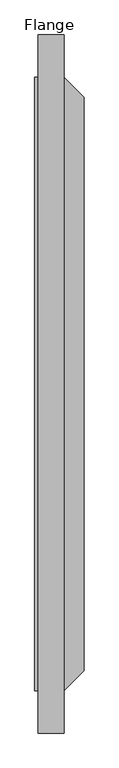
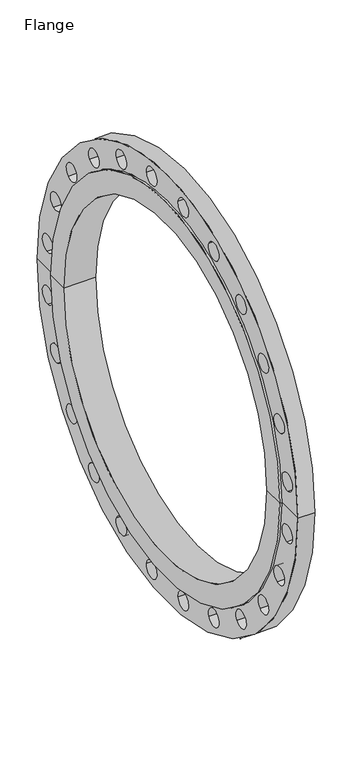
"""IFC4 building model written with IfcOpenShell, lengths in millimetres: proxy geometry, Flange : CASTED FLANGE PN16."""

import ifcopenshell
import ifcopenshell.guid

model = None  # the IFC model being written
_history = None  # IfcOwnerHistory: only IFC2X3 demands one
_inside = {}  # id of a spatial element -> (the spatial element, [elements in it])
_under = {}  # id of a project, library or spatial element -> (it, [spatial elements below it])
_declared = {}  # id of a project -> (the project, [libraries it declares])
_typed = {}  # id of a type object -> (the type object, [elements of that type])
_made_of = {}  # id of a material, layer set ... -> (it, [elements and type objects made of it])


def new_model(schema):
    """Start an empty IFC model of exactly this schema.

    Asked for "IFC4X3", IfcOpenShell would pick the latest addendum, in which some entities
    have other attributes; the version numbers below select the first issue.
    IFC2X3 requires an IfcOwnerHistory on every rooted entity: one is made here for all.
    """
    global model, _history
    if schema == "IFC4X3":
        model = ifcopenshell.file(schema_version=(4, 3, 0, 0))
    else:
        model = ifcopenshell.file(schema=schema)
    _inside.clear()
    _under.clear()
    _declared.clear()
    _typed.clear()
    _made_of.clear()
    _history = None
    if model.schema == "IFC2X3":
        org = make("IfcOrganization", Name="unknown")
        user = make(
            "IfcPersonAndOrganization",
            ThePerson=make("IfcPerson", FamilyName="unknown"),
            TheOrganization=org,
        )
        app = make(
            "IfcApplication",
            ApplicationDeveloper=org,
            Version="unknown",
            ApplicationFullName="unknown",
            ApplicationIdentifier="unknown",
        )
        _history = make(
            "IfcOwnerHistory",
            OwningUser=user,
            OwningApplication=app,
            ChangeAction="ADDED",
            CreationDate=0,
        )
    return model


def make(cls, **values):
    """One entity of the class cls with the attributes given. An attribute that is None is left unset."""
    return model.create_entity(
        cls, **{name: value for name, value in values.items() if value is not None}
    )


def rooted(cls, **values):
    """An entity with a GlobalId (a new one), such as an element, a storey or a relation."""
    return make(cls, GlobalId=ifcopenshell.guid.new(), OwnerHistory=_history, **values)


def si_unit(unit_type, name, prefix=None):
    """IfcSIUnit, for example si_unit("LENGTHUNIT", "METRE", prefix="MILLI")."""
    return make("IfcSIUnit", UnitType=unit_type, Prefix=prefix, Name=name)


def assignment(units):
    """IfcUnitAssignment: the units of a project."""
    return None if units is None else make("IfcUnitAssignment", Units=units)


def point(xyz):
    """IfcCartesianPoint."""
    return None if xyz is None else make("IfcCartesianPoint", Coordinates=xyz)


def direction(xyz):
    """IfcDirection."""
    return None if xyz is None else make("IfcDirection", DirectionRatios=xyz)


def frame(location, z_axis=None, x_axis=None):
    """IfcAxis2Placement3D, a coordinate frame: its origin and axes. An axis left out is left unset."""
    return make(
        "IfcAxis2Placement3D",
        Location=point(location),
        Axis=direction(z_axis),
        RefDirection=direction(x_axis),
    )


def origin():
    """The frame at (0, 0, 0) with its axes left unset."""
    return frame((0.0, 0.0, 0.0))


def place(relative_to, where):
    """IfcLocalPlacement: puts the frame where relative to a parent placement (None: the world)."""
    return make(
        "IfcLocalPlacement", PlacementRelTo=relative_to, RelativePlacement=where
    )


def context(
    kind, dimensions, precision=None, world=None, true_north=None, identifier=None
):
    """IfcGeometricRepresentationContext, for example the 3D "Model" context."""
    return make(
        "IfcGeometricRepresentationContext",
        ContextIdentifier=identifier,
        ContextType=kind,
        CoordinateSpaceDimension=dimensions,
        Precision=precision,
        WorldCoordinateSystem=world,
        TrueNorth=true_north,
    )


def project(units=None, contexts=None):
    """IfcProject with its units and contexts."""
    return rooted(
        "IfcProject",
        Name="project",
        RepresentationContexts=contexts,
        UnitsInContext=assignment(units),
    )


def spatial(cls, under=None, at=None, **own):
    """A site, building, storey or space (cls), placed at a placement, below another one or the project."""
    s = rooted(cls, ObjectPlacement=at, **own)
    if under is not None:
        _under.setdefault(under.id(), (under, []))[1].append(s)
    return s


def polyline(points):
    """IfcPolyline through the points."""
    return make("IfcPolyline", Points=[point(p) for p in points])


def circle_curve(where, radius):
    """IfcCircle in the frame where."""
    return make("IfcCircle", Position=where, Radius=radius)


def shape(context_of_items, identifier, shape_type, items):
    """IfcShapeRepresentation: the items that make up one representation, for example the "Body"."""
    return make(
        "IfcShapeRepresentation",
        ContextOfItems=context_of_items,
        RepresentationIdentifier=identifier,
        RepresentationType=shape_type,
        Items=items,
    )


def source(mapping_origin, context_of_items, identifier, shape_type, items):
    """IfcRepresentationMap: a shape defined once, which mapped items show again and again."""
    return make(
        "IfcRepresentationMap",
        MappingOrigin=mapping_origin,
        MappedRepresentation=shape(context_of_items, identifier, shape_type, items),
    )


def transform(
    local_origin,
    x_axis=None,
    y_axis=None,
    z_axis=None,
    scale=None,
    scale2=None,
    scale3=None,
    uniform=True,
):
    """IfcCartesianTransformationOperator3D, or its non-uniform kind. x_axis, y_axis, z_axis: its Axis1, 2, 3."""
    if uniform:
        return make(
            "IfcCartesianTransformationOperator3D",
            Axis1=direction(x_axis),
            Axis2=direction(y_axis),
            LocalOrigin=point(local_origin),
            Scale=scale,
            Axis3=direction(z_axis),
        )
    return make(
        "IfcCartesianTransformationOperator3DnonUniform",
        Axis1=direction(x_axis),
        Axis2=direction(y_axis),
        LocalOrigin=point(local_origin),
        Scale=scale,
        Axis3=direction(z_axis),
        Scale2=scale2,
        Scale3=scale3,
    )


def mapped(mapping_source, mapping_target):
    """IfcMappedItem: shows the shape of a source again, moved by a transform."""
    return make(
        "IfcMappedItem", MappingSource=mapping_source, MappingTarget=mapping_target
    )


def made_of(thing, what):
    """Note that an element or type object is made of a material, layer set ...; save() writes the relation."""
    if what is not None:
        _made_of.setdefault(what.id(), (what, []))[1].append(thing)
    return thing


def element(
    cls,
    number,
    at=None,
    inside=None,
    cuts=None,
    type_object=None,
    material=None,
    context=None,
    identifier="Body",
    shape_type=None,
    held_by="IfcProductDefinitionShape",
    body=None,
    shapes=None,
    **own,
):
    """One element of the class cls, such as IfcWall. Its Tag is "e" and its number.

    at: its placement. inside: the storey or other place that contains it. cuts: it is an
    opening in that element (IfcRelVoidsElement). A single representation is given by context,
    identifier, shape_type and body (its items); several are given by shapes. held_by: the class
    of the entity that holds the representations. save() writes the other relations.
    """
    e = rooted(cls, Tag="e%d" % number, ObjectPlacement=at, **own)
    if body is not None:
        shapes = [shape(context, identifier, shape_type, body)]
    if shapes is not None:
        e.Representation = make(held_by, Representations=shapes)
    if inside is not None:
        _inside.setdefault(inside.id(), (inside, []))[1].append(e)
    if cuts is not None:
        rooted(
            "IfcRelVoidsElement", RelatingBuildingElement=cuts, RelatedOpeningElement=e
        )
    if type_object is not None:
        _typed.setdefault(type_object.id(), (type_object, []))[1].append(e)
    return made_of(e, material)


def aggregate(whole, parts):
    """IfcRelAggregates: a whole, such as a stair, and the parts it consists of."""
    return rooted("IfcRelAggregates", RelatingObject=whole, RelatedObjects=parts)


def save(model, path):
    """Write the relations noted so far, then the file.

    IfcRelAggregates (storeys below a building ...), IfcRelContainedInSpatialStructure (elements
    in a storey), IfcRelDefinesByType, IfcRelAssociatesMaterial and IfcRelDeclares: one each for
    every whole, place, type object, material and project.
    """
    for whole, parts in _under.values():
        aggregate(whole, parts)
    for where, things in _inside.values():
        rooted(
            "IfcRelContainedInSpatialStructure",
            RelatedElements=things,
            RelatingStructure=where,
        )
    for kind, things in _typed.values():
        rooted("IfcRelDefinesByType", RelatedObjects=things, RelatingType=kind)
    for what, things in _made_of.values():
        rooted("IfcRelAssociatesMaterial", RelatedObjects=things, RelatingMaterial=what)
    for by, libraries in _declared.values():
        rooted("IfcRelDeclares", RelatingContext=by, RelatedDefinitions=libraries)
    model.write(path)


def plane_surface(at):
    """IfcPlane: the flat surface through the origin of the frame at, square to its z axis."""
    return make("IfcPlane", Position=at)


def cylinder_surface(at, radius):
    """IfcCylindricalSurface: all points at the distance radius from the z axis of the frame at."""
    return make("IfcCylindricalSurface", Position=at, Radius=radius)


def revolved_surface(curve, axis_point, axis_direction):
    """IfcSurfaceOfRevolution: the curve turned about the line through axis_point along axis_direction."""
    return make(
        "IfcSurfaceOfRevolution",
        SweptCurve=make("IfcArbitraryOpenProfileDef", ProfileType="CURVE", Curve=curve),
        AxisPosition=make("IfcAxis1Placement", Location=point(axis_point), Axis=direction(axis_direction)),
    )


def advanced_brep(points, edges, surfaces, faces):
    """IfcAdvancedBrep: a solid bounded by faces that lie on surfaces and meet in shared edges.

    An edge is (start, end): straight between two places in points (the first is 0);
    or (start, end, curve); or (start, end, curve, False) where it runs against its curve.
    A face is (place in surfaces, loops), or (place, loops, False) where it looks against
    its surface's normal. A loop lists edges by number (the first is 1), with a minus sign
    where the edge is run from its end to its start. The first loop is the outer one.
    """
    corners = [point(p) for p in points]
    vertices = [make("IfcVertexPoint", VertexGeometry=c) for c in corners]
    made = []
    for start, end, *more in edges:
        made.append(
            make(
                "IfcEdgeCurve",
                EdgeStart=vertices[start],
                EdgeEnd=vertices[end],
                EdgeGeometry=more[0] if more else make("IfcPolyline", Points=[corners[start], corners[end]]),
                SameSense=more[1] if len(more) > 1 else True,
            )
        )
    hull = []
    for where, loops, *sense in faces:
        bounds = []
        for j, loop in enumerate(loops):
            ring = [make("IfcOrientedEdge", EdgeElement=made[abs(k) - 1], Orientation=k > 0) for k in loop]
            bounds.append(
                make(
                    "IfcFaceOuterBound" if j == 0 else "IfcFaceBound",
                    Bound=make("IfcEdgeLoop", EdgeList=ring),
                    Orientation=True,
                )
            )
        hull.append(make("IfcAdvancedFace", Bounds=bounds, FaceSurface=surfaces[where], SameSense=sense[0] if sense else True))
    return make("IfcAdvancedBrep", Outer=make("IfcClosedShell", CfsFaces=hull))


def flange_f2916e97(model_context):
    return source(origin(), model_context, "Body", "AdvancedBrep", [
        advanced_brep(
        [(0.0, 400.0, 0.0), (0.0, 450.5, 0.0), (0.0, -450.5, 0.0), (0.0, -400.0, 0.0), (72.5, 400.0, 0.0), (72.5, -400.0, 0.0), (72.5, 421.0, 0.0), (72.5, -421.0, 0.0), (43.0, 450.5, 0.0), (43.0, -450.5, 0.0), (43.0, 512.5, 0.0), (43.0, -512.5, 0.0), (43.0, -82.324561, -468.2605222), (43.0, -41.6753216, -473.6120961), (43.0, 41.6753216, -473.6120961), (43.0, 82.324561, -468.2605222), (43.0, -200.7141608, -430.9977676), (43.0, -162.8351, -446.6877883), (43.0, -305.4254223, -364.3632273), (43.0, -272.8979353, -389.3224459), (43.0, -389.3224459, -272.8979353), (43.0, -364.3632273, -305.4254223), (43.0, -446.6877883, -162.8351), (43.0, -430.9977676, -200.7141608), (43.0, -473.6120961, -41.6753216), (43.0, -468.2605222, -82.324561), (43.0, 468.2605222, -82.324561), (43.0, 473.6120961, -41.6753216), (43.0, 272.8979353, -389.3224459), (43.0, 305.4254223, -364.3632273), (43.0, 162.8351, -446.6877883), (43.0, 200.7141608, -430.9977676), (43.0, 430.9977676, -200.7141608), (43.0, 446.6877883, -162.8351), (43.0, 364.3632273, -305.4254223), (43.0, 389.3224459, -272.8979353), (43.0, -468.2605222, 82.324561), (43.0, -473.6120961, 41.6753216), (43.0, -272.8979353, 389.3224459), (43.0, -305.4254223, 364.3632273), (43.0, -162.8351, 446.6877883), (43.0, -200.7141608, 430.9977676), (43.0, -41.6753216, 473.6120961), (43.0, -82.324561, 468.2605222), (43.0, 82.324561, 468.2605222), (43.0, 41.6753216, 473.6120961), (43.0, 200.7141608, 430.9977676), (43.0, 162.8351, 446.6877883), (43.0, 305.4254223, 364.3632273), (43.0, 272.8979353, 389.3224459), (43.0, 389.3224459, 272.8979353), (43.0, 364.3632273, 305.4254223), (43.0, 446.6877883, 162.8351), (43.0, 430.9977676, 200.7141608), (43.0, 473.6120961, 41.6753216), (43.0, 468.2605222, 82.324561), (43.0, -430.9977676, 200.7141608), (43.0, -446.6877883, 162.8351), (43.0, -364.3632273, 305.4254223), (43.0, -389.3224459, 272.8979353), (5.0, 512.5, 0.0), (5.0, -512.5, 0.0), (5.0, 450.5, 0.0), (5.0, -450.5, 0.0), (5.0, -41.6753216, -473.6120961), (5.0, -82.324561, -468.2605222), (5.0, 82.324561, -468.2605222), (5.0, 41.6753216, -473.6120961), (5.0, -162.8351, -446.6877883), (5.0, -200.7141608, -430.9977676), (5.0, -272.8979353, -389.3224459), (5.0, -305.4254223, -364.3632273), (5.0, -364.3632273, -305.4254223), (5.0, -389.3224459, -272.8979353), (5.0, -430.9977676, -200.7141608), (5.0, -446.6877883, -162.8351), (5.0, -468.2605222, -82.324561), (5.0, -473.6120961, -41.6753216), (5.0, 473.6120961, -41.6753216), (5.0, 468.2605222, -82.324561), (5.0, 305.4254223, -364.3632273), (5.0, 272.8979353, -389.3224459), (5.0, 200.7141608, -430.9977676), (5.0, 162.8351, -446.6877883), (5.0, 446.6877883, -162.8351), (5.0, 430.9977676, -200.7141608), (5.0, 389.3224459, -272.8979353), (5.0, 364.3632273, -305.4254223), (5.0, -473.6120961, 41.6753216), (5.0, -468.2605222, 82.324561), (5.0, -305.4254223, 364.3632273), (5.0, -272.8979353, 389.3224459), (5.0, -200.7141608, 430.9977676), (5.0, -162.8351, 446.6877883), (5.0, -82.324561, 468.2605222), (5.0, -41.6753216, 473.6120961), (5.0, 41.6753216, 473.6120961), (5.0, 82.324561, 468.2605222), (5.0, 162.8351, 446.6877883), (5.0, 200.7141608, 430.9977676), (5.0, 272.8979353, 389.3224459), (5.0, 305.4254223, 364.3632273), (5.0, 364.3632273, 305.4254223), (5.0, 389.3224459, 272.8979353), (5.0, 430.9977676, 200.7141608), (5.0, 446.6877883, 162.8351), (5.0, 468.2605222, 82.324561), (5.0, 473.6120961, 41.6753216), (5.0, -446.6877883, 162.8351), (5.0, -430.9977676, 200.7141608), (5.0, -389.3224459, 272.8979353), (5.0, -364.3632273, 305.4254223)],
        [
            (0, 1),
            (1, 2, circle_curve(frame((0.0, 0.0, 0.0), z_axis=(-1.0, 0.0, 0.0), x_axis=(0.0, 1.0, 0.0)), 450.5)),
            (2, 3),
            (3, 0, circle_curve(frame((0.0, 0.0, 0.0), z_axis=(1.0, 0.0, 0.0), x_axis=(0.0, 1.0, 0.0)), 400.0)),
            (0, 3, circle_curve(frame((0.0, 0.0, 0.0), z_axis=(1.0, 0.0, 0.0), x_axis=(0.0, 1.0, 0.0)), 400.0)),
            (2, 1, circle_curve(frame((0.0, 0.0, 0.0), z_axis=(-1.0, 0.0, 0.0), x_axis=(0.0, 1.0, 0.0)), 450.5)),
            (4, 0),
            (3, 5),
            (5, 4, circle_curve(frame((72.5, 0.0, 0.0), z_axis=(1.0, 0.0, 0.0), x_axis=(0.0, 1.0, 0.0)), 400.0)),
            (4, 5, circle_curve(frame((72.5, 0.0, 0.0), z_axis=(1.0, 0.0, 0.0), x_axis=(0.0, 1.0, 0.0)), 400.0)),
            (6, 4),
            (5, 7),
            (7, 6, circle_curve(frame((72.5, 0.0, 0.0), z_axis=(1.0, 0.0, 0.0), x_axis=(0.0, 1.0, 0.0)), 421.0)),
            (6, 7, circle_curve(frame((72.5, 0.0, 0.0), z_axis=(1.0, 0.0, 0.0), x_axis=(0.0, 1.0, 0.0)), 421.0)),
            (8, 6),
            (7, 9),
            (9, 8, circle_curve(frame((43.0, 0.0, 0.0), z_axis=(1.0, 0.0, 0.0), x_axis=(0.0, 1.0, 0.0)), 450.5)),
            (8, 9, circle_curve(frame((43.0, 0.0, 0.0), z_axis=(1.0, 0.0, 0.0), x_axis=(0.0, 1.0, 0.0)), 450.5)),
            (10, 8),
            (9, 11),
            (11, 10, circle_curve(frame((43.0, 0.0, 0.0), z_axis=(1.0, 0.0, 0.0), x_axis=(0.0, 1.0, 0.0)), 512.5)),
            (12, 13, circle_curve(frame((43.0, -61.9999413, -470.9363092), z_axis=(-1.0, 0.0, 0.0), x_axis=(0.0, 0.9914448613738129, -0.13052619222003253)), 20.5)),
            (13, 12, circle_curve(frame((43.0, -61.9999413, -470.9363092), z_axis=(-1.0, 0.0, 0.0), x_axis=(0.0, 0.9914448613738129, -0.13052619222003253)), 20.5)),
            (14, 15, circle_curve(frame((43.0, 61.9999413, -470.9363092), z_axis=(-1.0, 0.0, 0.0), x_axis=(0.0, 0.9914448613738089, 0.13052619222006298)), 20.5)),
            (15, 14, circle_curve(frame((43.0, 61.9999413, -470.9363092), z_axis=(-1.0, 0.0, 0.0), x_axis=(0.0, 0.9914448613738089, 0.13052619222006298)), 20.5)),
            (16, 17, circle_curve(frame((43.0, -181.7746304, -438.8427779), z_axis=(-1.0, 0.0, 0.0), x_axis=(0.0, 0.9238795325113015, -0.38268343236505475)), 20.5)),
            (17, 16, circle_curve(frame((43.0, -181.7746304, -438.8427779), z_axis=(-1.0, 0.0, 0.0), x_axis=(0.0, 0.9238795325113015, -0.38268343236505475)), 20.5)),
            (18, 19, circle_curve(frame((43.0, -289.1616788, -376.8428366), z_axis=(-1.0, 0.0, 0.0), x_axis=(0.0, 0.7933533402912514, -0.6087614290086997)), 20.5)),
            (19, 18, circle_curve(frame((43.0, -289.1616788, -376.8428366), z_axis=(-1.0, 0.0, 0.0), x_axis=(0.0, 0.7933533402912514, -0.6087614290086997)), 20.5)),
            (20, 21, circle_curve(frame((43.0, -376.8428366, -289.1616788), z_axis=(-1.0, 0.0, 0.0), x_axis=(0.0, 0.6087614290087368, -0.793353340291223)), 20.5)),
            (21, 20, circle_curve(frame((43.0, -376.8428366, -289.1616788), z_axis=(-1.0, 0.0, 0.0), x_axis=(0.0, 0.6087614290087368, -0.793353340291223)), 20.5)),
            (22, 23, circle_curve(frame((43.0, -438.8427779, -181.7746304), z_axis=(-1.0, 0.0, 0.0), x_axis=(0.0, 0.3826834323651087, -0.923879532511279)), 20.5)),
            (23, 22, circle_curve(frame((43.0, -438.8427779, -181.7746304), z_axis=(-1.0, 0.0, 0.0), x_axis=(0.0, 0.3826834323651087, -0.923879532511279)), 20.5)),
            (24, 25, circle_curve(frame((43.0, -470.9363092, -61.9999413), z_axis=(-1.0, 0.0, 0.0), x_axis=(0.0, 0.130526192220072, -0.9914448613738078)), 20.5)),
            (25, 24, circle_curve(frame((43.0, -470.9363092, -61.9999413), z_axis=(-1.0, 0.0, 0.0), x_axis=(0.0, 0.130526192220072, -0.9914448613738078)), 20.5)),
            (26, 27, circle_curve(frame((43.0, 470.9363092, -61.9999413), z_axis=(-1.0, 0.0, 0.0), x_axis=(0.0, 0.13052619222001557, 0.9914448613738153)), 20.5)),
            (27, 26, circle_curve(frame((43.0, 470.9363092, -61.9999413), z_axis=(-1.0, 0.0, 0.0), x_axis=(0.0, 0.13052619222001557, 0.9914448613738153)), 20.5)),
            (28, 29, circle_curve(frame((43.0, 289.1616788, -376.8428366), z_axis=(-1.0, 0.0, 0.0), x_axis=(0.0, 0.7933533402912125, 0.6087614290087502)), 20.5)),
            (29, 28, circle_curve(frame((43.0, 289.1616788, -376.8428366), z_axis=(-1.0, 0.0, 0.0), x_axis=(0.0, 0.7933533402912125, 0.6087614290087502)), 20.5)),
            (30, 31, circle_curve(frame((43.0, 181.7746304, -438.8427779), z_axis=(-1.0, 0.0, 0.0), x_axis=(0.0, 0.9238795325112725, 0.3826834323651245)), 20.5)),
            (31, 30, circle_curve(frame((43.0, 181.7746304, -438.8427779), z_axis=(-1.0, 0.0, 0.0), x_axis=(0.0, 0.9238795325112725, 0.3826834323651245)), 20.5)),
            (32, 33, circle_curve(frame((43.0, 438.8427779, -181.7746304), z_axis=(-1.0, 0.0, 0.0), x_axis=(0.0, 0.38268343236505586, 0.9238795325113008)), 20.5)),
            (33, 32, circle_curve(frame((43.0, 438.8427779, -181.7746304), z_axis=(-1.0, 0.0, 0.0), x_axis=(0.0, 0.38268343236505586, 0.9238795325113008)), 20.5)),
            (34, 35, circle_curve(frame((43.0, 376.8428366, -289.1616788), z_axis=(-1.0, 0.0, 0.0), x_axis=(0.0, 0.6087614290086916, 0.7933533402912578)), 20.5)),
            (35, 34, circle_curve(frame((43.0, 376.8428366, -289.1616788), z_axis=(-1.0, 0.0, 0.0), x_axis=(0.0, 0.6087614290086916, 0.7933533402912578)), 20.5)),
            (10, 11, circle_curve(frame((43.0, 0.0, 0.0), z_axis=(1.0, 0.0, 0.0), x_axis=(0.0, 1.0, 0.0)), 512.5)),
            (36, 37, circle_curve(frame((43.0, -470.9363092, 61.9999413), z_axis=(-1.0, 0.0, 0.0), x_axis=(0.0, -0.13052619222003067, -0.9914448613738133)), 20.5)),
            (37, 36, circle_curve(frame((43.0, -470.9363092, 61.9999413), z_axis=(-1.0, 0.0, 0.0), x_axis=(0.0, -0.13052619222003067, -0.9914448613738133)), 20.5)),
            (38, 39, circle_curve(frame((43.0, -289.1616788, 376.8428366), z_axis=(-1.0, 0.0, 0.0), x_axis=(0.0, -0.7933533402912221, -0.6087614290087378)), 20.5)),
            (39, 38, circle_curve(frame((43.0, -289.1616788, 376.8428366), z_axis=(-1.0, 0.0, 0.0), x_axis=(0.0, -0.7933533402912221, -0.6087614290087378)), 20.5)),
            (40, 41, circle_curve(frame((43.0, -181.7746304, 438.8427779), z_axis=(-1.0, 0.0, 0.0), x_axis=(0.0, -0.9238795325112785, -0.38268343236510993)), 20.5)),
            (41, 40, circle_curve(frame((43.0, -181.7746304, 438.8427779), z_axis=(-1.0, 0.0, 0.0), x_axis=(0.0, -0.9238795325112785, -0.38268343236510993)), 20.5)),
            (42, 43, circle_curve(frame((43.0, -61.9999413, 470.9363092), z_axis=(-1.0, 0.0, 0.0), x_axis=(0.0, -0.9914448613738076, -0.1305261922200736)), 20.5)),
            (43, 42, circle_curve(frame((43.0, -61.9999413, 470.9363092), z_axis=(-1.0, 0.0, 0.0), x_axis=(0.0, -0.9914448613738076, -0.1305261922200736)), 20.5)),
            (44, 45, circle_curve(frame((43.0, 61.9999413, 470.9363092), z_axis=(-1.0, 0.0, 0.0), x_axis=(0.0, -0.9914448613738134, 0.13052619222002934)), 20.5)),
            (45, 44, circle_curve(frame((43.0, 61.9999413, 470.9363092), z_axis=(-1.0, 0.0, 0.0), x_axis=(0.0, -0.9914448613738134, 0.13052619222002934)), 20.5)),
            (46, 47, circle_curve(frame((43.0, 181.7746304, 438.8427779), z_axis=(-1.0, 0.0, 0.0), x_axis=(0.0, -0.9238795325113007, 0.3826834323650564)), 20.5)),
            (47, 46, circle_curve(frame((43.0, 181.7746304, 438.8427779), z_axis=(-1.0, 0.0, 0.0), x_axis=(0.0, -0.9238795325113007, 0.3826834323650564)), 20.5)),
            (48, 49, circle_curve(frame((43.0, 289.1616788, 376.8428366), z_axis=(-1.0, 0.0, 0.0), x_axis=(0.0, -0.7933533402912568, 0.6087614290086926)), 20.5)),
            (49, 48, circle_curve(frame((43.0, 289.1616788, 376.8428366), z_axis=(-1.0, 0.0, 0.0), x_axis=(0.0, -0.7933533402912568, 0.6087614290086926)), 20.5)),
            (50, 51, circle_curve(frame((43.0, 376.8428366, 289.1616788), z_axis=(-1.0, 0.0, 0.0), x_axis=(0.0, -0.6087614290087492, 0.7933533402912134)), 20.5)),
            (51, 50, circle_curve(frame((43.0, 376.8428366, 289.1616788), z_axis=(-1.0, 0.0, 0.0), x_axis=(0.0, -0.6087614290087492, 0.7933533402912134)), 20.5)),
            (52, 53, circle_curve(frame((43.0, 438.8427779, 181.7746304), z_axis=(-1.0, 0.0, 0.0), x_axis=(0.0, -0.38268343236512353, 0.923879532511273)), 20.5)),
            (53, 52, circle_curve(frame((43.0, 438.8427779, 181.7746304), z_axis=(-1.0, 0.0, 0.0), x_axis=(0.0, -0.38268343236512353, 0.923879532511273)), 20.5)),
            (54, 55, circle_curve(frame((43.0, 470.9363092, 61.9999413), z_axis=(-1.0, 0.0, 0.0), x_axis=(0.0, -0.13052619222008732, 0.9914448613738058)), 20.5)),
            (55, 54, circle_curve(frame((43.0, 470.9363092, 61.9999413), z_axis=(-1.0, 0.0, 0.0), x_axis=(0.0, -0.13052619222008732, 0.9914448613738058)), 20.5)),
            (56, 57, circle_curve(frame((43.0, -438.8427779, 181.7746304), z_axis=(-1.0, 0.0, 0.0), x_axis=(0.0, -0.3826834323650704, -0.9238795325112948)), 20.5)),
            (57, 56, circle_curve(frame((43.0, -438.8427779, 181.7746304), z_axis=(-1.0, 0.0, 0.0), x_axis=(0.0, -0.3826834323650704, -0.9238795325112948)), 20.5)),
            (58, 59, circle_curve(frame((43.0, -376.8428366, 289.1616788), z_axis=(-1.0, 0.0, 0.0), x_axis=(0.0, -0.6087614290087036, -0.7933533402912484)), 20.5)),
            (59, 58, circle_curve(frame((43.0, -376.8428366, 289.1616788), z_axis=(-1.0, 0.0, 0.0), x_axis=(0.0, -0.6087614290087036, -0.7933533402912484)), 20.5)),
            (60, 10),
            (11, 61),
            (61, 60, circle_curve(frame((5.0, 0.0, 0.0), z_axis=(1.0, 0.0, 0.0), x_axis=(0.0, 1.0, 0.0)), 512.5)),
            (60, 61, circle_curve(frame((5.0, 0.0, 0.0), z_axis=(1.0, 0.0, 0.0), x_axis=(0.0, 1.0, 0.0)), 512.5)),
            (62, 60),
            (61, 63),
            (63, 62, circle_curve(frame((5.0, 0.0, 0.0), z_axis=(1.0, 0.0, 0.0), x_axis=(0.0, 1.0, 0.0)), 450.5)),
            (64, 65, circle_curve(frame((5.0, -61.9999413, -470.9363092), z_axis=(1.0, 0.0, 0.0), x_axis=(0.0, 0.9914448613738129, -0.13052619222003253)), 20.5)),
            (65, 64, circle_curve(frame((5.0, -61.9999413, -470.9363092), z_axis=(1.0, 0.0, 0.0), x_axis=(0.0, 0.9914448613738129, -0.13052619222003253)), 20.5)),
            (66, 67, circle_curve(frame((5.0, 61.9999413, -470.9363092), z_axis=(1.0, 0.0, 0.0), x_axis=(0.0, 0.9914448613738089, 0.13052619222006298)), 20.5)),
            (67, 66, circle_curve(frame((5.0, 61.9999413, -470.9363092), z_axis=(1.0, 0.0, 0.0), x_axis=(0.0, 0.9914448613738089, 0.13052619222006298)), 20.5)),
            (68, 69, circle_curve(frame((5.0, -181.7746304, -438.8427779), z_axis=(1.0, 0.0, 0.0), x_axis=(0.0, 0.9238795325113015, -0.38268343236505475)), 20.5)),
            (69, 68, circle_curve(frame((5.0, -181.7746304, -438.8427779), z_axis=(1.0, 0.0, 0.0), x_axis=(0.0, 0.9238795325113015, -0.38268343236505475)), 20.5)),
            (70, 71, circle_curve(frame((5.0, -289.1616788, -376.8428366), z_axis=(1.0, 0.0, 0.0), x_axis=(0.0, 0.7933533402912514, -0.6087614290086997)), 20.5)),
            (71, 70, circle_curve(frame((5.0, -289.1616788, -376.8428366), z_axis=(1.0, 0.0, 0.0), x_axis=(0.0, 0.7933533402912514, -0.6087614290086997)), 20.5)),
            (72, 73, circle_curve(frame((5.0, -376.8428366, -289.1616788), z_axis=(1.0, 0.0, 0.0), x_axis=(0.0, 0.6087614290087368, -0.793353340291223)), 20.5)),
            (73, 72, circle_curve(frame((5.0, -376.8428366, -289.1616788), z_axis=(1.0, 0.0, 0.0), x_axis=(0.0, 0.6087614290087368, -0.793353340291223)), 20.5)),
            (74, 75, circle_curve(frame((5.0, -438.8427779, -181.7746304), z_axis=(1.0, 0.0, 0.0), x_axis=(0.0, 0.3826834323651087, -0.923879532511279)), 20.5)),
            (75, 74, circle_curve(frame((5.0, -438.8427779, -181.7746304), z_axis=(1.0, 0.0, 0.0), x_axis=(0.0, 0.3826834323651087, -0.923879532511279)), 20.5)),
            (76, 77, circle_curve(frame((5.0, -470.9363092, -61.9999413), z_axis=(1.0, 0.0, 0.0), x_axis=(0.0, 0.130526192220072, -0.9914448613738078)), 20.5)),
            (77, 76, circle_curve(frame((5.0, -470.9363092, -61.9999413), z_axis=(1.0, 0.0, 0.0), x_axis=(0.0, 0.130526192220072, -0.9914448613738078)), 20.5)),
            (78, 79, circle_curve(frame((5.0, 470.9363092, -61.9999413), z_axis=(1.0, 0.0, 0.0), x_axis=(0.0, 0.13052619222001557, 0.9914448613738153)), 20.5)),
            (79, 78, circle_curve(frame((5.0, 470.9363092, -61.9999413), z_axis=(1.0, 0.0, 0.0), x_axis=(0.0, 0.13052619222001557, 0.9914448613738153)), 20.5)),
            (80, 81, circle_curve(frame((5.0, 289.1616788, -376.8428366), z_axis=(1.0, 0.0, 0.0), x_axis=(0.0, 0.7933533402912125, 0.6087614290087502)), 20.5)),
            (81, 80, circle_curve(frame((5.0, 289.1616788, -376.8428366), z_axis=(1.0, 0.0, 0.0), x_axis=(0.0, 0.7933533402912125, 0.6087614290087502)), 20.5)),
            (82, 83, circle_curve(frame((5.0, 181.7746304, -438.8427779), z_axis=(1.0, 0.0, 0.0), x_axis=(0.0, 0.9238795325112725, 0.3826834323651245)), 20.5)),
            (83, 82, circle_curve(frame((5.0, 181.7746304, -438.8427779), z_axis=(1.0, 0.0, 0.0), x_axis=(0.0, 0.9238795325112725, 0.3826834323651245)), 20.5)),
            (84, 85, circle_curve(frame((5.0, 438.8427779, -181.7746304), z_axis=(1.0, 0.0, 0.0), x_axis=(0.0, 0.38268343236505586, 0.9238795325113008)), 20.5)),
            (85, 84, circle_curve(frame((5.0, 438.8427779, -181.7746304), z_axis=(1.0, 0.0, 0.0), x_axis=(0.0, 0.38268343236505586, 0.9238795325113008)), 20.5)),
            (86, 87, circle_curve(frame((5.0, 376.8428366, -289.1616788), z_axis=(1.0, 0.0, 0.0), x_axis=(0.0, 0.6087614290086916, 0.7933533402912578)), 20.5)),
            (87, 86, circle_curve(frame((5.0, 376.8428366, -289.1616788), z_axis=(1.0, 0.0, 0.0), x_axis=(0.0, 0.6087614290086916, 0.7933533402912578)), 20.5)),
            (62, 63, circle_curve(frame((5.0, 0.0, 0.0), z_axis=(1.0, 0.0, 0.0), x_axis=(0.0, 1.0, 0.0)), 450.5)),
            (88, 89, circle_curve(frame((5.0, -470.9363092, 61.9999413), z_axis=(1.0, 0.0, 0.0), x_axis=(0.0, -0.13052619222003067, -0.9914448613738133)), 20.5)),
            (89, 88, circle_curve(frame((5.0, -470.9363092, 61.9999413), z_axis=(1.0, 0.0, 0.0), x_axis=(0.0, -0.13052619222003067, -0.9914448613738133)), 20.5)),
            (90, 91, circle_curve(frame((5.0, -289.1616788, 376.8428366), z_axis=(1.0, 0.0, 0.0), x_axis=(0.0, -0.7933533402912221, -0.6087614290087378)), 20.5)),
            (91, 90, circle_curve(frame((5.0, -289.1616788, 376.8428366), z_axis=(1.0, 0.0, 0.0), x_axis=(0.0, -0.7933533402912221, -0.6087614290087378)), 20.5)),
            (92, 93, circle_curve(frame((5.0, -181.7746304, 438.8427779), z_axis=(1.0, 0.0, 0.0), x_axis=(0.0, -0.9238795325112785, -0.38268343236510993)), 20.5)),
            (93, 92, circle_curve(frame((5.0, -181.7746304, 438.8427779), z_axis=(1.0, 0.0, 0.0), x_axis=(0.0, -0.9238795325112785, -0.38268343236510993)), 20.5)),
            (94, 95, circle_curve(frame((5.0, -61.9999413, 470.9363092), z_axis=(1.0, 0.0, 0.0), x_axis=(0.0, -0.9914448613738076, -0.1305261922200736)), 20.5)),
            (95, 94, circle_curve(frame((5.0, -61.9999413, 470.9363092), z_axis=(1.0, 0.0, 0.0), x_axis=(0.0, -0.9914448613738076, -0.1305261922200736)), 20.5)),
            (96, 97, circle_curve(frame((5.0, 61.9999413, 470.9363092), z_axis=(1.0, 0.0, 0.0), x_axis=(0.0, -0.9914448613738134, 0.13052619222002934)), 20.5)),
            (97, 96, circle_curve(frame((5.0, 61.9999413, 470.9363092), z_axis=(1.0, 0.0, 0.0), x_axis=(0.0, -0.9914448613738134, 0.13052619222002934)), 20.5)),
            (98, 99, circle_curve(frame((5.0, 181.7746304, 438.8427779), z_axis=(1.0, 0.0, 0.0), x_axis=(0.0, -0.9238795325113007, 0.3826834323650564)), 20.5)),
            (99, 98, circle_curve(frame((5.0, 181.7746304, 438.8427779), z_axis=(1.0, 0.0, 0.0), x_axis=(0.0, -0.9238795325113007, 0.3826834323650564)), 20.5)),
            (100, 101, circle_curve(frame((5.0, 289.1616788, 376.8428366), z_axis=(1.0, 0.0, 0.0), x_axis=(0.0, -0.7933533402912568, 0.6087614290086926)), 20.5)),
            (101, 100, circle_curve(frame((5.0, 289.1616788, 376.8428366), z_axis=(1.0, 0.0, 0.0), x_axis=(0.0, -0.7933533402912568, 0.6087614290086926)), 20.5)),
            (102, 103, circle_curve(frame((5.0, 376.8428366, 289.1616788), z_axis=(1.0, 0.0, 0.0), x_axis=(0.0, -0.6087614290087492, 0.7933533402912134)), 20.5)),
            (103, 102, circle_curve(frame((5.0, 376.8428366, 289.1616788), z_axis=(1.0, 0.0, 0.0), x_axis=(0.0, -0.6087614290087492, 0.7933533402912134)), 20.5)),
            (104, 105, circle_curve(frame((5.0, 438.8427779, 181.7746304), z_axis=(1.0, 0.0, 0.0), x_axis=(0.0, -0.38268343236512353, 0.923879532511273)), 20.5)),
            (105, 104, circle_curve(frame((5.0, 438.8427779, 181.7746304), z_axis=(1.0, 0.0, 0.0), x_axis=(0.0, -0.38268343236512353, 0.923879532511273)), 20.5)),
            (106, 107, circle_curve(frame((5.0, 470.9363092, 61.9999413), z_axis=(1.0, 0.0, 0.0), x_axis=(0.0, -0.13052619222008732, 0.9914448613738058)), 20.5)),
            (107, 106, circle_curve(frame((5.0, 470.9363092, 61.9999413), z_axis=(1.0, 0.0, 0.0), x_axis=(0.0, -0.13052619222008732, 0.9914448613738058)), 20.5)),
            (108, 109, circle_curve(frame((5.0, -438.8427779, 181.7746304), z_axis=(1.0, 0.0, 0.0), x_axis=(0.0, -0.3826834323650704, -0.9238795325112948)), 20.5)),
            (109, 108, circle_curve(frame((5.0, -438.8427779, 181.7746304), z_axis=(1.0, 0.0, 0.0), x_axis=(0.0, -0.3826834323650704, -0.9238795325112948)), 20.5)),
            (110, 111, circle_curve(frame((5.0, -376.8428366, 289.1616788), z_axis=(1.0, 0.0, 0.0), x_axis=(0.0, -0.6087614290087036, -0.7933533402912484)), 20.5)),
            (111, 110, circle_curve(frame((5.0, -376.8428366, 289.1616788), z_axis=(1.0, 0.0, 0.0), x_axis=(0.0, -0.6087614290087036, -0.7933533402912484)), 20.5)),
            (1, 62),
            (63, 2),
            (12, 65),
            (64, 13),
            (14, 67),
            (66, 15),
            (16, 69),
            (68, 17),
            (18, 71),
            (70, 19),
            (20, 73),
            (72, 21),
            (22, 75),
            (74, 23),
            (24, 77),
            (76, 25),
            (36, 89),
            (88, 37),
            (56, 109),
            (108, 57),
            (58, 111),
            (110, 59),
            (38, 91),
            (90, 39),
            (40, 93),
            (92, 41),
            (42, 95),
            (94, 43),
            (44, 97),
            (96, 45),
            (46, 99),
            (98, 47),
            (48, 101),
            (100, 49),
            (50, 103),
            (102, 51),
            (52, 105),
            (104, 53),
            (54, 107),
            (106, 55),
            (26, 79),
            (78, 27),
            (32, 85),
            (84, 33),
            (34, 87),
            (86, 35),
            (28, 81),
            (80, 29),
            (30, 83),
            (82, 31),
        ],
        [
            plane_surface(frame((0.0, 0.0, 0.0), z_axis=(-1.0, 0.0, 0.0), x_axis=(0.0, 1.0, 0.0))),
            revolved_surface(polyline([(0.0, 400.0, 0.0), (72.5, 400.0, 0.0)]), (-95.0, 0.0, 0.0), (-1.0, 0.0, 0.0)),
            plane_surface(frame((72.5, 0.0, 0.0), z_axis=(1.0, 0.0, 0.0), x_axis=(0.0, 1.0, 0.0))),
            revolved_surface(polyline([(72.5, 421.0, 0.0), (43.0, 450.5, 0.0)]), (-95.0, 0.0, 0.0), (-1.0, 0.0, 0.0)),
            plane_surface(frame((43.0, 0.0, 0.0), z_axis=(1.0, 0.0, 0.0), x_axis=(0.0, 1.0, 0.0))),
            cylinder_surface(frame((-95.0, 0.0, 0.0), z_axis=(-1.0, 0.0, 0.0), x_axis=(0.0, 1.0, 0.0)), 512.5),
            plane_surface(frame((5.0, 0.0, 0.0), z_axis=(-1.0, 0.0, 0.0), x_axis=(0.0, 1.0, 0.0))),
            cylinder_surface(frame((-95.0, 0.0, 0.0), z_axis=(-1.0, 0.0, 0.0), x_axis=(0.0, 1.0, 0.0)), 450.5),
            revolved_surface(polyline([(5.0, -41.67532164183684, -473.61209614051063), (43.0, -41.67532164183684, -473.61209614051063)]), (43.0, -61.9999413, -470.9363092), (-1.0, 0.0, 0.0)),
            revolved_surface(polyline([(5.0, 82.32456095816309, -468.2605222594887), (43.0, 82.32456095816309, -468.2605222594887)]), (43.0, 61.9999413, -470.9363092), (-1.0, 0.0, 0.0)),
            revolved_surface(polyline([(4.999999999999986, -162.83509998351832, -446.6877882634836), (43.0, -162.83509998351832, -446.6877882634836)]), (43.0, -181.7746304, -438.8427779), (-1.0000000000000002, 0.0, 0.0)),
            revolved_surface(polyline([(5.0, -272.89793532402933, -389.32244589467837), (43.0, -272.89793532402933, -389.32244589467837)]), (43.0, -289.1616788, -376.8428366), (-1.0, 0.0, 0.0)),
            revolved_surface(polyline([(4.999999999999986, -364.3632273053209, -305.42542227597005), (43.0, -364.3632273053209, -305.42542227597005)]), (43.0, -376.8428366, -289.1616788), (-1.0000000000000002, 0.0, 0.0)),
            revolved_surface(polyline([(5.0, -430.99776753651525, -200.71416081648124), (43.0, -430.99776753651525, -200.71416081648124)]), (43.0, -438.8427779, -181.7746304), (-1.0, 0.0, 0.0)),
            revolved_surface(polyline([(5.0, -468.2605222594885, -82.32456095816306), (43.0, -468.2605222594885, -82.32456095816306)]), (43.0, -470.9363092, -61.9999413), (-1.0, 0.0, 0.0)),
            revolved_surface(polyline([(5.0, -473.61209614051063, 41.67532164183683), (43.0, -473.61209614051063, 41.67532164183683)]), (43.0, -470.9363092, 61.9999413), (-1.0, 0.0, 0.0)),
            revolved_surface(polyline([(5.0, -446.6877882634839, 162.83509998351846), (43.0, -446.6877882634839, 162.83509998351846)]), (43.0, -438.8427779, 181.7746304), (-1.0, 0.0, 0.0)),
            revolved_surface(polyline([(5.0, -389.3224458946784, 272.8979353240294), (43.0, -389.3224458946784, 272.8979353240294)]), (43.0, -376.8428366, 289.1616788), (-1.0, 0.0, 0.0)),
            revolved_surface(polyline([(5.0, -305.42542227597005, 364.3632273053209), (43.0, -305.42542227597005, 364.3632273053209)]), (43.0, -289.1616788, 376.8428366), (-1.0, 0.0, 0.0)),
            revolved_surface(polyline([(5.0, -200.7141608164812, 430.99776753651525), (43.0, -200.7141608164812, 430.99776753651525)]), (43.0, -181.7746304, 438.8427779), (-1.0, 0.0, 0.0)),
            revolved_surface(polyline([(4.999999999999986, -82.32456095816306, 468.2605222594885), (43.0, -82.32456095816306, 468.2605222594885)]), (43.0, -61.9999413, 470.9363092), (-1.0000000000000002, 0.0, 0.0)),
            revolved_surface(polyline([(5.0, 41.67532164183683, 473.6120961405106), (43.0, 41.67532164183683, 473.6120961405106)]), (43.0, 61.9999413, 470.9363092), (-1.0, 0.0, 0.0)),
            revolved_surface(polyline([(5.0, 162.83509998351835, 446.68778826348364), (43.0, 162.83509998351835, 446.68778826348364)]), (43.0, 181.7746304, 438.8427779), (-1.0, 0.0, 0.0)),
            revolved_surface(polyline([(5.0, 272.8979353240292, 389.3224458946782), (43.0, 272.8979353240292, 389.3224458946782)]), (43.0, 289.1616788, 376.8428366), (-1.0, 0.0, 0.0)),
            revolved_surface(polyline([(5.0, 364.36322730532066, 305.4254222759699), (43.0, 364.36322730532066, 305.4254222759699)]), (43.0, 376.8428366, 289.1616788), (-1.0, 0.0, 0.0)),
            revolved_surface(polyline([(5.0, 430.99776753651497, 200.7141608164811), (43.0, 430.99776753651497, 200.7141608164811)]), (43.0, 438.8427779, 181.7746304), (-1.0, 0.0, 0.0)),
            revolved_surface(polyline([(4.999999999999986, 468.2605222594882, 82.32456095816302), (43.0, 468.2605222594882, 82.32456095816302)]), (43.0, 470.9363092, 61.9999413), (-1.0000000000000002, 0.0, 0.0)),
            revolved_surface(polyline([(5.0, 473.6120961405103, -41.67532164183679), (43.0, 473.6120961405103, -41.67532164183679)]), (43.0, 470.9363092, -61.9999413), (-1.0, 0.0, 0.0)),
            revolved_surface(polyline([(5.0, 446.68778826348364, -162.83509998351835), (43.0, 446.68778826348364, -162.83509998351835)]), (43.0, 438.8427779, -181.7746304), (-1.0, 0.0, 0.0)),
            revolved_surface(polyline([(4.999999999999986, 389.3224458946782, -272.8979353240292), (43.0, 389.3224458946782, -272.8979353240292)]), (43.0, 376.8428366, -289.1616788), (-1.0000000000000002, 0.0, 0.0)),
            revolved_surface(polyline([(5.0, 305.4254222759699, -364.3632273053206), (43.0, 305.4254222759699, -364.3632273053206)]), (43.0, 289.1616788, -376.8428366), (-1.0, 0.0, 0.0)),
            revolved_surface(polyline([(5.0, 200.7141608164811, -430.9977675365149), (43.0, 200.7141608164811, -430.9977675365149)]), (43.0, 181.7746304, -438.8427779), (-1.0, 0.0, 0.0)),
        ],
        [
            (0, [[1, 2, 3, 4]]),
            (0, [[-1, 5, -3, 6]]),
            (1, [[7, -4, 8, 9]]),
            (1, [[-7, 10, -8, -5]]),
            (2, [[11, -9, 12, 13]]),
            (2, [[-11, 14, -12, -10]]),
            (3, [[15, -13, 16, 17]]),
            (3, [[-15, 18, -16, -14]]),
            (4, [[19, -17, 20, 21], [22, 23], [24, 25], [26, 27], [28, 29], [30, 31], [32, 33], [34, 35], [36, 37], [38, 39], [40, 41], [42, 43], [44, 45]]),
            (4, [[-19, 46, -20, -18], [47, 48], [49, 50], [51, 52], [53, 54], [55, 56], [57, 58], [59, 60], [61, 62], [63, 64], [65, 66], [67, 68], [69, 70]]),
            (5, [[71, -21, 72, 73]]),
            (5, [[-71, 74, -72, -46]]),
            (6, [[75, -73, 76, 77], [78, 79], [80, 81], [82, 83], [84, 85], [86, 87], [88, 89], [90, 91], [92, 93], [94, 95], [96, 97], [98, 99], [100, 101]]),
            (6, [[-75, 102, -76, -74], [103, 104], [105, 106], [107, 108], [109, 110], [111, 112], [113, 114], [115, 116], [117, 118], [119, 120], [121, 122], [123, 124], [125, 126]]),
            (7, [[127, -77, 128, -2]]),
            (7, [[-127, -6, -128, -102]]),
            (8, [[129, -78, 130, -22]]),
            (8, [[-129, -23, -130, -79]]),
            (9, [[131, -80, 132, -24]]),
            (9, [[-131, -25, -132, -81]]),
            (10, [[133, -82, 134, -26]]),
            (10, [[-133, -27, -134, -83]]),
            (11, [[135, -84, 136, -28]]),
            (11, [[-135, -29, -136, -85]]),
            (12, [[137, -86, 138, -30]]),
            (12, [[-137, -31, -138, -87]]),
            (13, [[139, -88, 140, -32]]),
            (13, [[-139, -33, -140, -89]]),
            (14, [[141, -90, 142, -34]]),
            (14, [[-141, -35, -142, -91]]),
            (15, [[143, -103, 144, -47]]),
            (15, [[-143, -48, -144, -104]]),
            (16, [[145, -123, 146, -67]]),
            (16, [[-145, -68, -146, -124]]),
            (17, [[147, -125, 148, -69]]),
            (17, [[-147, -70, -148, -126]]),
            (18, [[149, -105, 150, -49]]),
            (18, [[-149, -50, -150, -106]]),
            (19, [[151, -107, 152, -51]]),
            (19, [[-151, -52, -152, -108]]),
            (20, [[153, -109, 154, -53]]),
            (20, [[-153, -54, -154, -110]]),
            (21, [[155, -111, 156, -55]]),
            (21, [[-155, -56, -156, -112]]),
            (22, [[157, -113, 158, -57]]),
            (22, [[-157, -58, -158, -114]]),
            (23, [[159, -115, 160, -59]]),
            (23, [[-159, -60, -160, -116]]),
            (24, [[161, -117, 162, -61]]),
            (24, [[-161, -62, -162, -118]]),
            (25, [[163, -119, 164, -63]]),
            (25, [[-163, -64, -164, -120]]),
            (26, [[165, -121, 166, -65]]),
            (26, [[-165, -66, -166, -122]]),
            (27, [[167, -92, 168, -36]]),
            (27, [[-167, -37, -168, -93]]),
            (28, [[169, -98, 170, -42]]),
            (28, [[-169, -43, -170, -99]]),
            (29, [[171, -100, 172, -44]]),
            (29, [[-171, -45, -172, -101]]),
            (30, [[173, -94, 174, -38]]),
            (30, [[-173, -39, -174, -95]]),
            (31, [[175, -96, 176, -40]]),
            (31, [[-175, -41, -176, -97]]),
        ],
    ),
    ])


if __name__ == "__main__":
    model = new_model("IFC4")
    model_context = context("Model", 3, world=origin())
    ifc_project = project(units=[si_unit("LENGTHUNIT", "METRE", prefix="MILLI")], contexts=[model_context])
    site = spatial("IfcSite", under=ifc_project)
    building = spatial("IfcBuilding", under=site)
    placement = place(None, origin())
    flange_shape = flange_f2916e97(model_context)
    element("IfcBuildingElementProxy", 1, Name="Flange : CASTED FLANGE PN16", ObjectType="Flange : CASTED FLANGE PN16", at=placement, inside=building, context=model_context, shape_type="MappedRepresentation", body=[
        mapped(flange_shape, transform((0.0, 0.0, 0.0), x_axis=(1.0, 0.0, 0.0), y_axis=(0.0, 1.0, 0.0), z_axis=(0.0, 0.0, 1.0))),
    ])
    save(model, "model.ifc")

# Revit data of these elements
# Type "Flange : CASTED FLANGE PN16"
#   TABLE_DIMENSIONS = "DIMENSIONS FIXED FLANGE"
#   Short Description = ""
#   Description = "FIXED FLANGE"
#   K [instance default] = 110 mm
#   HOLE DIAMETER [instance default] = 19 mm
#   D4 [instance default] = 84 mm
#   DRILL DIAMETER [instance default] = 110 mm
#   DN [instance default] = 40 mm
#   D2 [instance default] = 70 mm
#   D [instance default] = 150 mm
#   f [instance default] = 3 mm
#   b [instance default] = 16 mm
#   ANGLE [instance default] = 45.00°
#   a [instance default] = 19 mm
#   PN = 16
#   BOLTS NUMBER [instance default] = 4
#   MATERIAL [instance default] = none
#   COATING [instance default] = none
#   Default Elevation = 0
# Element 1 (IfcBuildingElementProxy, "Flange : CASTED FLANGE PN16")
#   K = 950 mm
#   HOLE DIAMETER = 41 mm
#   D4 = 901 mm
#   DRILL DIAMETER = 950 mm
#   DN = 800 mm
#   D2 = 842 mm
#   D = 1025 mm
#   f = 5 mm
#   b = 38 mm
#   a = 43 mm
#   BOLTS NUMBER = 24
#   COATING = Not informed
#   Materials on its faces: "Not informed"
# Materials
#   "Not informed": class "Paint/Coating", colour RGB 0 56 123, transparency 0, Description = "Not Informed", Cost = 0
